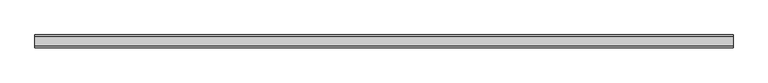
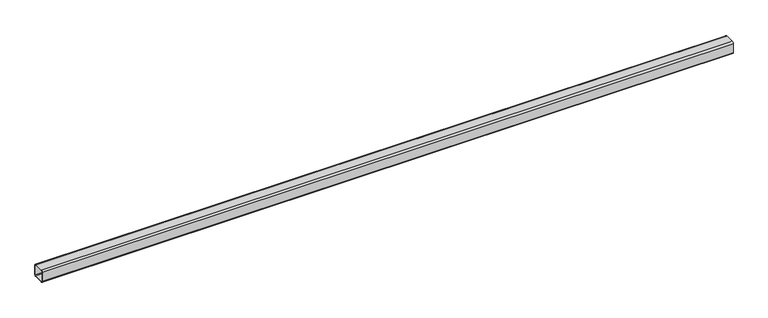
"""IFC4 building model written with IfcOpenShell, lengths in millimetres: beam geometry, Гнутый прямоугольный профиль (Трубы 30245-94) Балки : гнутый прямоуг. проф. 100x6."""

from ifc_helpers import new_model, si_unit, point, frame, frame_2d, origin, place, context, project, spatial, polyline, circle_curve, trimmed, segment, composite_curve, outline, extrude, source, transform, mapped, element, save


def beam_eb9d9f0c(model_context):
    return source(origin(), model_context, "Body", "SweptSolid", [
        extrude(outline(composite_curve([segment(polyline([(-38.0, 50.0), (38.0, 50.0)]), True, "CONTINUOUS"), segment(trimmed(circle_curve(frame_2d((38.0, 38.0)), 12.0), [point((38.0, 50.0))], [point((50.0, 38.0))], False, "CARTESIAN"), True, "CONTINUOUS"), segment(polyline([(50.0, 38.0), (50.0, -38.0)]), True, "CONTINUOUS"), segment(trimmed(circle_curve(frame_2d((38.0, -38.0)), 12.0), [point((50.0, -38.0))], [point((38.0, -50.0))], False, "CARTESIAN"), True, "CONTINUOUS"), segment(polyline([(38.0, -50.0), (-38.0, -50.0)]), True, "CONTINUOUS"), segment(trimmed(circle_curve(frame_2d((-38.0, -38.0)), 12.0), [point((-38.0, -50.0))], [point((-50.0, -38.0))], False, "CARTESIAN"), True, "CONTINUOUS"), segment(polyline([(-50.0, -38.0), (-50.0, 38.0)]), True, "CONTINUOUS"), segment(trimmed(circle_curve(frame_2d((-38.0, 38.0)), 12.0), [point((-50.0, 38.0))], [point((-38.0, 50.0))], False, "CARTESIAN"), True, "CONTINUOUS")], self_intersect=False), holes=[composite_curve([segment(trimmed(circle_curve(frame_2d((-38.0, 38.0)), 6.0), [point((-38.0, 44.0))], [point((-44.0, 38.0))], True, "CARTESIAN"), True, "CONTINUOUS"), segment(polyline([(-44.0, 38.0), (-44.0, -38.0)]), True, "CONTINUOUS"), segment(trimmed(circle_curve(frame_2d((-38.0, -38.0)), 6.0), [point((-44.0, -38.0))], [point((-38.0, -44.0))], True, "CARTESIAN"), True, "CONTINUOUS"), segment(polyline([(-38.0, -44.0), (38.0, -44.0)]), True, "CONTINUOUS"), segment(trimmed(circle_curve(frame_2d((38.0, -38.0)), 6.0), [point((38.0, -44.0))], [point((44.0, -38.0))], True, "CARTESIAN"), True, "CONTINUOUS"), segment(polyline([(44.0, -38.0), (44.0, 38.0)]), True, "CONTINUOUS"), segment(trimmed(circle_curve(frame_2d((38.0, 38.0)), 6.0), [point((44.0, 38.0))], [point((38.0, 44.0))], True, "CARTESIAN"), True, "CONTINUOUS"), segment(polyline([(38.0, 44.0), (-38.0, 44.0)]), True, "CONTINUOUS")], self_intersect=False)]), frame((-2750.0, 0.0, 0.0), z_axis=(1.0, 0.0, 0.0), x_axis=(0.0, 1.0, 0.0)), (0.0, 0.0, 1.0), 5500.0),
    ])


if __name__ == "__main__":
    model = new_model("IFC4")
    model_context = context("Model", 3, world=origin())
    ifc_project = project(units=[si_unit("LENGTHUNIT", "METRE", prefix="MILLI")], contexts=[model_context])
    site = spatial("IfcSite", under=ifc_project)
    building = spatial("IfcBuilding", under=site)
    placement = place(None, origin())
    beam_shape = beam_eb9d9f0c(model_context)
    element("IfcBeam", 1, ObjectType="Гнутый прямоугольный профиль (Трубы 30245-94) Балки : гнутый прямоуг. проф. 100x6", at=placement, inside=building, context=model_context, shape_type="MappedRepresentation", body=[
        mapped(beam_shape, transform((0.0, 0.0, 0.0), x_axis=(1.0, 0.0, 0.0), y_axis=(0.0, 1.0, 0.0), z_axis=(0.0, 0.0, 1.0))),
    ])
    save(model, "model.ifc")

# Revit data of these elements
# Type "Гнутый прямоугольный профиль (Трубы 30245-94) Балки : гнутый прямоуг. проф. 100x6"
#   ri = 12 mm
#   ra = 6 mm
#   W = 0.173578
#   Vz = 50 mm
#   Vy = 50 mm
#   Vpz = 50 mm
#   Vpy = 50 mm
#   Length [instance default] = 1500 mm
#   bf = 100 mm
#   d = 100 mm
#   tf = 6 mm
#   tw = 6 mm
#   A = 0.00226 m²
#   Structural Material [instance default] = Металл - Сталь - 345 МПa
#   Assembly Code = ""
# Element 1 (IfcBeam, "Гнутый прямоугольный профиль (Трубы 30245-94) Балки : гнутый прямоуг. проф. 100x6")
#   Structural Material = C235
#   Materials on its faces: "C235"
# Materials
#   "Металл - Сталь - 345 МПa": class "Металл", colour RGB 247 247 247, transparency 0
#   "C235": class "Не назначено", colour RGB 0 0 0, transparency 0
